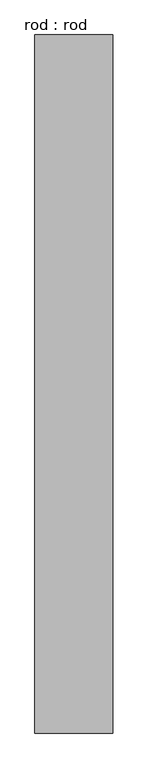
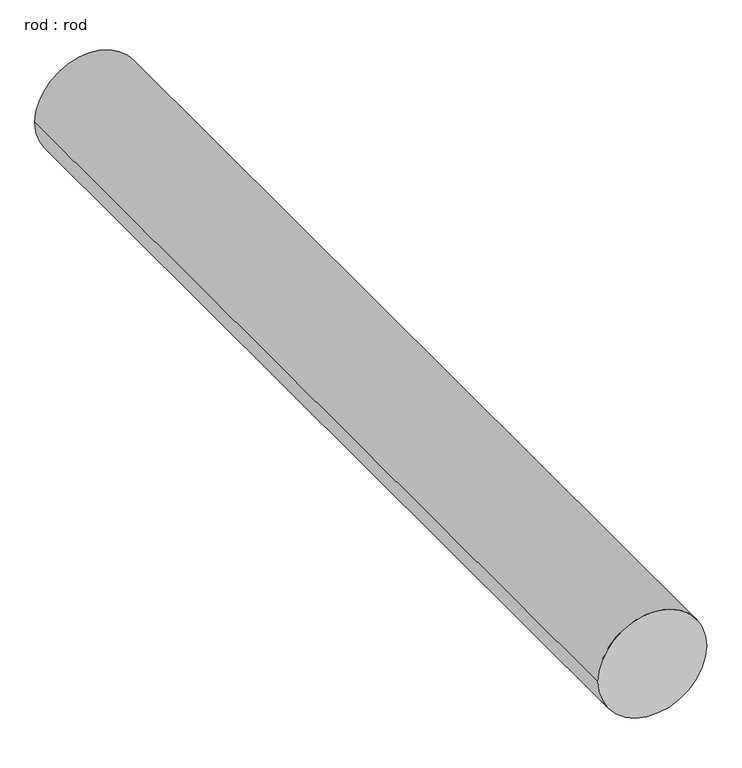
"""IFC4 building model written with IfcOpenShell, lengths in millimetres: proxy geometry, rod : rod."""

from ifc_helpers import new_model, si_unit, point, frame, frame_2d, origin, place, context, project, spatial, circle_curve, trimmed, segment, composite_curve, outline, extrude, source, transform, mapped, element, save


def rod_rod_7ab98d1f(model_context):
    return source(origin(), model_context, "Body", "SweptSolid", [
        extrude(outline(composite_curve([segment(trimmed(circle_curve(frame_2d((0.0108462, 0.0)), 200.0), [point((0.0108462, 200.0))], [point((0.0108462, -200.0))], False, "CARTESIAN"), True, "CONTINUOUS"), segment(trimmed(circle_curve(frame_2d((0.0108462, 0.0)), 200.0), [point((0.0108462, -200.0))], [point((0.0108462, 200.0))], False, "CARTESIAN"), True, "CONTINUOUS")], self_intersect=False)), frame((0.0, 2299.4756354, 0.0), z_axis=(0.0, 1.0, 0.0), x_axis=(0.0, 0.0, 1.0)), (0.0, 0.0, 1.0), 3586.5059598),
    ])


if __name__ == "__main__":
    model = new_model("IFC4")
    model_context = context("Model", 3, world=origin())
    ifc_project = project(units=[si_unit("LENGTHUNIT", "METRE", prefix="MILLI")], contexts=[model_context])
    site = spatial("IfcSite", under=ifc_project)
    building = spatial("IfcBuilding", under=site)
    placement = place(None, origin())
    rod_rod_shape = rod_rod_7ab98d1f(model_context)
    element("IfcBuildingElementProxy", 1, Name="rod : rod", ObjectType="rod : rod", at=placement, inside=building, context=model_context, shape_type="MappedRepresentation", body=[
        mapped(rod_rod_shape, transform((0.0, 0.0, 0.0), x_axis=(1.0, 0.0, 0.0), y_axis=(0.0, 1.0, 0.0), z_axis=(0.0, 0.0, 1.0))),
    ])
    save(model, "model.ifc")

# Revit data of these elements
# Type "rod : rod"
#   Default Elevation = 0
